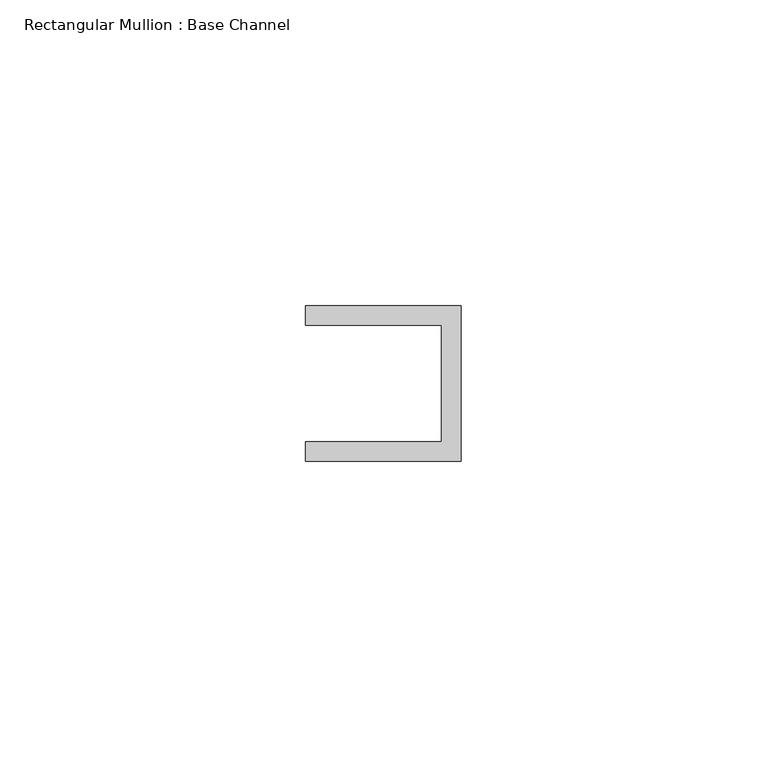
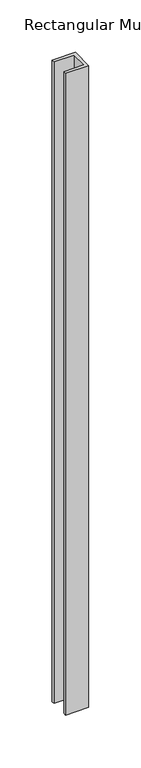
"""IFC4 building model written with IfcOpenShell, lengths in millimetres: member geometry, Rectangular Mullion : Base Channel."""

import ifcopenshell
import ifcopenshell.guid

model = None  # the IFC model being written
_history = None  # IfcOwnerHistory: only IFC2X3 demands one
_inside = {}  # id of a spatial element -> (the spatial element, [elements in it])
_under = {}  # id of a project, library or spatial element -> (it, [spatial elements below it])
_declared = {}  # id of a project -> (the project, [libraries it declares])
_typed = {}  # id of a type object -> (the type object, [elements of that type])
_made_of = {}  # id of a material, layer set ... -> (it, [elements and type objects made of it])


def new_model(schema):
    """Start an empty IFC model of exactly this schema.

    Asked for "IFC4X3", IfcOpenShell would pick the latest addendum, in which some entities
    have other attributes; the version numbers below select the first issue.
    IFC2X3 requires an IfcOwnerHistory on every rooted entity: one is made here for all.
    """
    global model, _history
    if schema == "IFC4X3":
        model = ifcopenshell.file(schema_version=(4, 3, 0, 0))
    else:
        model = ifcopenshell.file(schema=schema)
    _inside.clear()
    _under.clear()
    _declared.clear()
    _typed.clear()
    _made_of.clear()
    _history = None
    if model.schema == "IFC2X3":
        org = make("IfcOrganization", Name="unknown")
        user = make(
            "IfcPersonAndOrganization",
            ThePerson=make("IfcPerson", FamilyName="unknown"),
            TheOrganization=org,
        )
        app = make(
            "IfcApplication",
            ApplicationDeveloper=org,
            Version="unknown",
            ApplicationFullName="unknown",
            ApplicationIdentifier="unknown",
        )
        _history = make(
            "IfcOwnerHistory",
            OwningUser=user,
            OwningApplication=app,
            ChangeAction="ADDED",
            CreationDate=0,
        )
    return model


def make(cls, **values):
    """One entity of the class cls with the attributes given. An attribute that is None is left unset."""
    return model.create_entity(
        cls, **{name: value for name, value in values.items() if value is not None}
    )


def rooted(cls, **values):
    """An entity with a GlobalId (a new one), such as an element, a storey or a relation."""
    return make(cls, GlobalId=ifcopenshell.guid.new(), OwnerHistory=_history, **values)


def si_unit(unit_type, name, prefix=None):
    """IfcSIUnit, for example si_unit("LENGTHUNIT", "METRE", prefix="MILLI")."""
    return make("IfcSIUnit", UnitType=unit_type, Prefix=prefix, Name=name)


def assignment(units):
    """IfcUnitAssignment: the units of a project."""
    return None if units is None else make("IfcUnitAssignment", Units=units)


def point(xyz):
    """IfcCartesianPoint."""
    return None if xyz is None else make("IfcCartesianPoint", Coordinates=xyz)


def direction(xyz):
    """IfcDirection."""
    return None if xyz is None else make("IfcDirection", DirectionRatios=xyz)


def frame(location, z_axis=None, x_axis=None):
    """IfcAxis2Placement3D, a coordinate frame: its origin and axes. An axis left out is left unset."""
    return make(
        "IfcAxis2Placement3D",
        Location=point(location),
        Axis=direction(z_axis),
        RefDirection=direction(x_axis),
    )


def origin():
    """The frame at (0, 0, 0) with its axes left unset."""
    return frame((0.0, 0.0, 0.0))


def place(relative_to, where):
    """IfcLocalPlacement: puts the frame where relative to a parent placement (None: the world)."""
    return make(
        "IfcLocalPlacement", PlacementRelTo=relative_to, RelativePlacement=where
    )


def context(
    kind, dimensions, precision=None, world=None, true_north=None, identifier=None
):
    """IfcGeometricRepresentationContext, for example the 3D "Model" context."""
    return make(
        "IfcGeometricRepresentationContext",
        ContextIdentifier=identifier,
        ContextType=kind,
        CoordinateSpaceDimension=dimensions,
        Precision=precision,
        WorldCoordinateSystem=world,
        TrueNorth=true_north,
    )


def project(units=None, contexts=None):
    """IfcProject with its units and contexts."""
    return rooted(
        "IfcProject",
        Name="project",
        RepresentationContexts=contexts,
        UnitsInContext=assignment(units),
    )


def spatial(cls, under=None, at=None, **own):
    """A site, building, storey or space (cls), placed at a placement, below another one or the project."""
    s = rooted(cls, ObjectPlacement=at, **own)
    if under is not None:
        _under.setdefault(under.id(), (under, []))[1].append(s)
    return s


def polyline(points):
    """IfcPolyline through the points."""
    return make("IfcPolyline", Points=[point(p) for p in points])


def outline(outer, holes=None, kind="AREA"):
    """IfcArbitraryClosedProfileDef: a profile drawn as a closed curve; with holes, ...WithVoids."""
    if holes is None:
        return make("IfcArbitraryClosedProfileDef", ProfileType=kind, OuterCurve=outer)
    return make(
        "IfcArbitraryProfileDefWithVoids",
        ProfileType=kind,
        OuterCurve=outer,
        InnerCurves=holes,
    )


def extrude(swept, where, along, depth):
    """IfcExtrudedAreaSolid: the profile swept, set in the frame where, extruded along a direction by depth."""
    return make(
        "IfcExtrudedAreaSolid",
        SweptArea=swept,
        Position=where,
        ExtrudedDirection=direction(along),
        Depth=depth,
    )


def shape(context_of_items, identifier, shape_type, items):
    """IfcShapeRepresentation: the items that make up one representation, for example the "Body"."""
    return make(
        "IfcShapeRepresentation",
        ContextOfItems=context_of_items,
        RepresentationIdentifier=identifier,
        RepresentationType=shape_type,
        Items=items,
    )


def source(mapping_origin, context_of_items, identifier, shape_type, items):
    """IfcRepresentationMap: a shape defined once, which mapped items show again and again."""
    return make(
        "IfcRepresentationMap",
        MappingOrigin=mapping_origin,
        MappedRepresentation=shape(context_of_items, identifier, shape_type, items),
    )


def transform(
    local_origin,
    x_axis=None,
    y_axis=None,
    z_axis=None,
    scale=None,
    scale2=None,
    scale3=None,
    uniform=True,
):
    """IfcCartesianTransformationOperator3D, or its non-uniform kind. x_axis, y_axis, z_axis: its Axis1, 2, 3."""
    if uniform:
        return make(
            "IfcCartesianTransformationOperator3D",
            Axis1=direction(x_axis),
            Axis2=direction(y_axis),
            LocalOrigin=point(local_origin),
            Scale=scale,
            Axis3=direction(z_axis),
        )
    return make(
        "IfcCartesianTransformationOperator3DnonUniform",
        Axis1=direction(x_axis),
        Axis2=direction(y_axis),
        LocalOrigin=point(local_origin),
        Scale=scale,
        Axis3=direction(z_axis),
        Scale2=scale2,
        Scale3=scale3,
    )


def mapped(mapping_source, mapping_target):
    """IfcMappedItem: shows the shape of a source again, moved by a transform."""
    return make(
        "IfcMappedItem", MappingSource=mapping_source, MappingTarget=mapping_target
    )


def made_of(thing, what):
    """Note that an element or type object is made of a material, layer set ...; save() writes the relation."""
    if what is not None:
        _made_of.setdefault(what.id(), (what, []))[1].append(thing)
    return thing


def element(
    cls,
    number,
    at=None,
    inside=None,
    cuts=None,
    type_object=None,
    material=None,
    context=None,
    identifier="Body",
    shape_type=None,
    held_by="IfcProductDefinitionShape",
    body=None,
    shapes=None,
    **own,
):
    """One element of the class cls, such as IfcWall. Its Tag is "e" and its number.

    at: its placement. inside: the storey or other place that contains it. cuts: it is an
    opening in that element (IfcRelVoidsElement). A single representation is given by context,
    identifier, shape_type and body (its items); several are given by shapes. held_by: the class
    of the entity that holds the representations. save() writes the other relations.
    """
    e = rooted(cls, Tag="e%d" % number, ObjectPlacement=at, **own)
    if body is not None:
        shapes = [shape(context, identifier, shape_type, body)]
    if shapes is not None:
        e.Representation = make(held_by, Representations=shapes)
    if inside is not None:
        _inside.setdefault(inside.id(), (inside, []))[1].append(e)
    if cuts is not None:
        rooted(
            "IfcRelVoidsElement", RelatingBuildingElement=cuts, RelatedOpeningElement=e
        )
    if type_object is not None:
        _typed.setdefault(type_object.id(), (type_object, []))[1].append(e)
    return made_of(e, material)


def aggregate(whole, parts):
    """IfcRelAggregates: a whole, such as a stair, and the parts it consists of."""
    return rooted("IfcRelAggregates", RelatingObject=whole, RelatedObjects=parts)


def save(model, path):
    """Write the relations noted so far, then the file.

    IfcRelAggregates (storeys below a building ...), IfcRelContainedInSpatialStructure (elements
    in a storey), IfcRelDefinesByType, IfcRelAssociatesMaterial and IfcRelDeclares: one each for
    every whole, place, type object, material and project.
    """
    for whole, parts in _under.values():
        aggregate(whole, parts)
    for where, things in _inside.values():
        rooted(
            "IfcRelContainedInSpatialStructure",
            RelatedElements=things,
            RelatingStructure=where,
        )
    for kind, things in _typed.values():
        rooted("IfcRelDefinesByType", RelatedObjects=things, RelatingType=kind)
    for what, things in _made_of.values():
        rooted("IfcRelAssociatesMaterial", RelatedObjects=things, RelatingMaterial=what)
    for by, libraries in _declared.values():
        rooted("IfcRelDeclares", RelatingContext=by, RelatedDefinitions=libraries)
    model.write(path)


def rectangular_mullion_base_channel_aef695ff(model_context):
    return source(origin(), model_context, "Body", "SweptSolid", [
        extrude(outline(polyline([(0.0, -12.7), (-25.4, -12.7), (-25.4, -9.525), (-3.175, -9.525), (-3.175, 9.525), (-25.4, 9.525), (-25.4, 12.7), (0.0, 12.7), (0.0, -12.7)])), frame((0.0, 0.0, -747.1996433), z_axis=(0.0, 0.0, 1.0), x_axis=(1.0, 0.0, 0.0)), (0.0, 0.0, 1.0), 747.1996433),
    ])


if __name__ == "__main__":
    model = new_model("IFC4")
    model_context = context("Model", 3, world=origin())
    ifc_project = project(units=[si_unit("LENGTHUNIT", "METRE", prefix="MILLI")], contexts=[model_context])
    site = spatial("IfcSite", under=ifc_project)
    building = spatial("IfcBuilding", under=site)
    placement = place(None, origin())
    rectangular_mullion_base_channel_shape = rectangular_mullion_base_channel_aef695ff(model_context)
    element("IfcMember", 1, ObjectType="Rectangular Mullion : Base Channel", at=placement, inside=building, context=model_context, shape_type="MappedRepresentation", body=[
        mapped(rectangular_mullion_base_channel_shape, transform((0.0, 0.0, 0.0), x_axis=(1.0, 0.0, 0.0), y_axis=(0.0, 1.0, 0.0), z_axis=(0.0, 0.0, 1.0))),
    ])
    save(model, "model.ifc")

# Revit data of these elements
# Type "Rectangular Mullion : Base Channel"
#   built-in parameter 1007322 = 0.0833333 (stored number, unit not read)
#   built-in parameter 1007321 = 0.0416667 (stored number, unit not read)
#   built-in parameter 1007320 = -0.03125 (stored number, unit not read)
# Element 1 (IfcMember, "Rectangular Mullion : Base Channel")
#   Materials on its faces: "ALUM"
# Materials
#   "ALUM": class "Generic", colour RGB 157 157 157, transparency 0, Cost = 0
